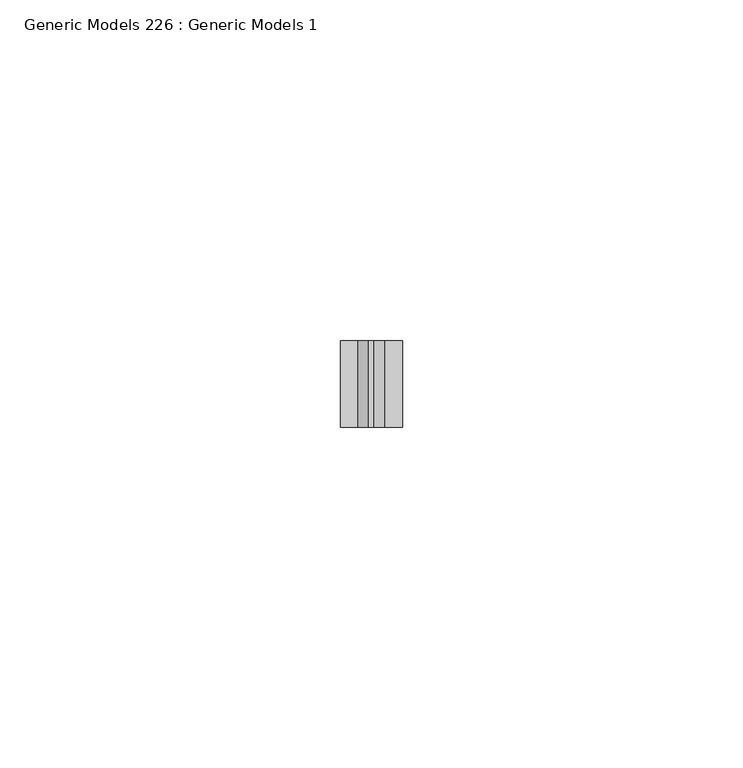
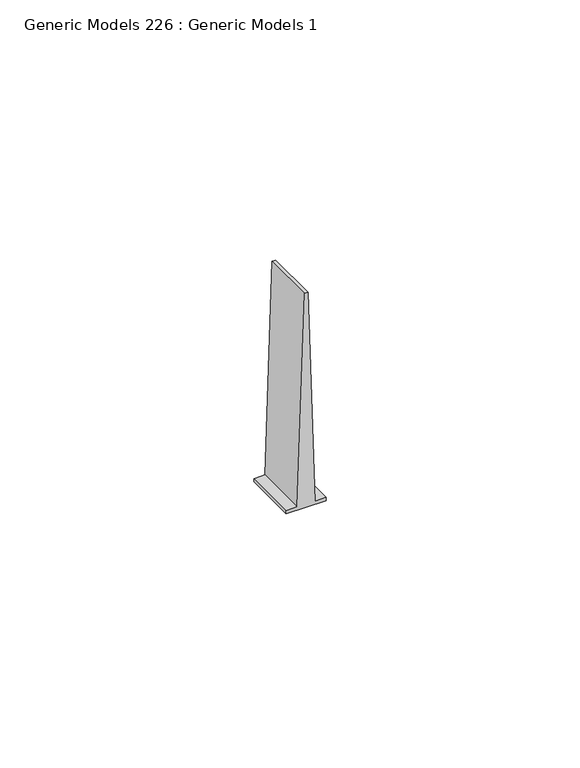
"""IFC4 building model written with IfcOpenShell, lengths in millimetres: proxy geometry, Generic Models 226 : Generic Models 1."""

from ifc_helpers import new_model, si_unit, frame, origin, place, context, project, spatial, polyline, outline, extrude, source, transform, mapped, element, save


def generic_models_226_generic_models_1_ff61dcbf(model_context):
    return source(origin(), model_context, "Body", "SweptSolid", [
        extrude(outline(polyline([(3338.9089294, 52599.8605108), (3338.9089294, 52608.9537108), (3339.7026794, 52608.9537108), (3339.7026794, 52606.4038472), (3390.5026794, 52604.8064581), (3390.5026794, 52604.0077635), (3339.7026794, 52602.4103744), (3339.7026794, 52599.8605108), (3338.9089294, 52599.8605108)])), frame((0.0, 565.15, 0.0), z_axis=(0.0, 1.0, 0.0), x_axis=(0.0, 0.0, 1.0)), (0.0, 0.0, 1.0), 12.7),
    ])


if __name__ == "__main__":
    model = new_model("IFC4")
    model_context = context("Model", 3, world=origin())
    ifc_project = project(units=[si_unit("LENGTHUNIT", "METRE", prefix="MILLI")], contexts=[model_context])
    site = spatial("IfcSite", under=ifc_project)
    building = spatial("IfcBuilding", under=site)
    placement = place(None, origin())
    generic_models_226_generic_models_1_shape = generic_models_226_generic_models_1_ff61dcbf(model_context)
    element("IfcBuildingElementProxy", 1, Name="Generic Models 226 : Generic Models 1", ObjectType="Generic Models 226 : Generic Models 1", at=placement, inside=building, context=model_context, shape_type="MappedRepresentation", body=[
        mapped(generic_models_226_generic_models_1_shape, transform((0.0, 0.0, 0.0), x_axis=(1.0, 0.0, 0.0), y_axis=(0.0, 1.0, 0.0), z_axis=(0.0, 0.0, 1.0))),
    ])
    save(model, "model.ifc")

# Revit data of these elements
# Element 1 (IfcBuildingElementProxy, "Generic Models 226 : Generic Models 1")
#   Materials on its faces: "METAL RUNNER CHANNEL; FASTEN @ 24\" O.C."
# Materials
#   "METAL RUNNER CHANNEL; FASTEN @ 24\" O.C.": class "Unassigned", colour RGB 210 209 208, transparency 0, Keynote = "M05121300.02", Cost = 0
